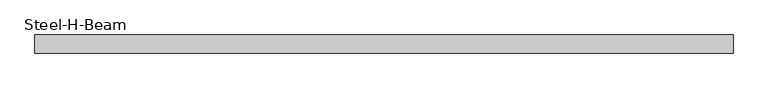
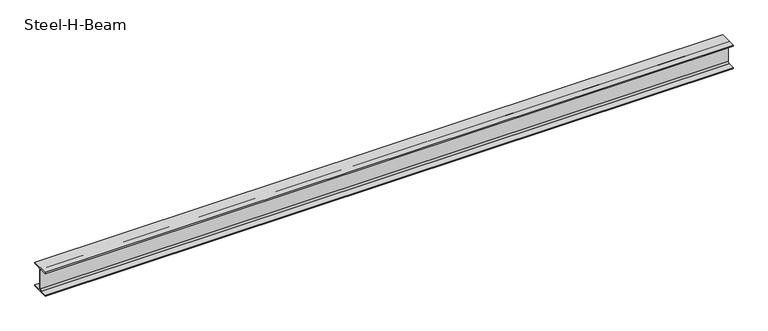
"""IFC4 building model written with IfcOpenShell, lengths in millimetres: beam geometry, Steel-H-Beam : BM121_H-244×175x7x11."""

import ifcopenshell
import ifcopenshell.guid

model = None  # the IFC model being written
_history = None  # IfcOwnerHistory: only IFC2X3 demands one
_inside = {}  # id of a spatial element -> (the spatial element, [elements in it])
_under = {}  # id of a project, library or spatial element -> (it, [spatial elements below it])
_declared = {}  # id of a project -> (the project, [libraries it declares])
_typed = {}  # id of a type object -> (the type object, [elements of that type])
_made_of = {}  # id of a material, layer set ... -> (it, [elements and type objects made of it])


def new_model(schema):
    """Start an empty IFC model of exactly this schema.

    Asked for "IFC4X3", IfcOpenShell would pick the latest addendum, in which some entities
    have other attributes; the version numbers below select the first issue.
    IFC2X3 requires an IfcOwnerHistory on every rooted entity: one is made here for all.
    """
    global model, _history
    if schema == "IFC4X3":
        model = ifcopenshell.file(schema_version=(4, 3, 0, 0))
    else:
        model = ifcopenshell.file(schema=schema)
    _inside.clear()
    _under.clear()
    _declared.clear()
    _typed.clear()
    _made_of.clear()
    _history = None
    if model.schema == "IFC2X3":
        org = make("IfcOrganization", Name="unknown")
        user = make(
            "IfcPersonAndOrganization",
            ThePerson=make("IfcPerson", FamilyName="unknown"),
            TheOrganization=org,
        )
        app = make(
            "IfcApplication",
            ApplicationDeveloper=org,
            Version="unknown",
            ApplicationFullName="unknown",
            ApplicationIdentifier="unknown",
        )
        _history = make(
            "IfcOwnerHistory",
            OwningUser=user,
            OwningApplication=app,
            ChangeAction="ADDED",
            CreationDate=0,
        )
    return model


def make(cls, **values):
    """One entity of the class cls with the attributes given. An attribute that is None is left unset."""
    return model.create_entity(
        cls, **{name: value for name, value in values.items() if value is not None}
    )


def rooted(cls, **values):
    """An entity with a GlobalId (a new one), such as an element, a storey or a relation."""
    return make(cls, GlobalId=ifcopenshell.guid.new(), OwnerHistory=_history, **values)


def si_unit(unit_type, name, prefix=None):
    """IfcSIUnit, for example si_unit("LENGTHUNIT", "METRE", prefix="MILLI")."""
    return make("IfcSIUnit", UnitType=unit_type, Prefix=prefix, Name=name)


def assignment(units):
    """IfcUnitAssignment: the units of a project."""
    return None if units is None else make("IfcUnitAssignment", Units=units)


def point(xyz):
    """IfcCartesianPoint."""
    return None if xyz is None else make("IfcCartesianPoint", Coordinates=xyz)


def direction(xyz):
    """IfcDirection."""
    return None if xyz is None else make("IfcDirection", DirectionRatios=xyz)


def frame(location, z_axis=None, x_axis=None):
    """IfcAxis2Placement3D, a coordinate frame: its origin and axes. An axis left out is left unset."""
    return make(
        "IfcAxis2Placement3D",
        Location=point(location),
        Axis=direction(z_axis),
        RefDirection=direction(x_axis),
    )


def frame_2d(location, x_axis=None):
    """IfcAxis2Placement2D, a coordinate frame in the plane: its origin and x axis."""
    return make(
        "IfcAxis2Placement2D", Location=point(location), RefDirection=direction(x_axis)
    )


def origin():
    """The frame at (0, 0, 0) with its axes left unset."""
    return frame((0.0, 0.0, 0.0))


def place(relative_to, where):
    """IfcLocalPlacement: puts the frame where relative to a parent placement (None: the world)."""
    return make(
        "IfcLocalPlacement", PlacementRelTo=relative_to, RelativePlacement=where
    )


def context(
    kind, dimensions, precision=None, world=None, true_north=None, identifier=None
):
    """IfcGeometricRepresentationContext, for example the 3D "Model" context."""
    return make(
        "IfcGeometricRepresentationContext",
        ContextIdentifier=identifier,
        ContextType=kind,
        CoordinateSpaceDimension=dimensions,
        Precision=precision,
        WorldCoordinateSystem=world,
        TrueNorth=true_north,
    )


def project(units=None, contexts=None):
    """IfcProject with its units and contexts."""
    return rooted(
        "IfcProject",
        Name="project",
        RepresentationContexts=contexts,
        UnitsInContext=assignment(units),
    )


def spatial(cls, under=None, at=None, **own):
    """A site, building, storey or space (cls), placed at a placement, below another one or the project."""
    s = rooted(cls, ObjectPlacement=at, **own)
    if under is not None:
        _under.setdefault(under.id(), (under, []))[1].append(s)
    return s


def polyline(points):
    """IfcPolyline through the points."""
    return make("IfcPolyline", Points=[point(p) for p in points])


def circle_curve(where, radius):
    """IfcCircle in the frame where."""
    return make("IfcCircle", Position=where, Radius=radius)


def trimmed(basis, trim1, trim2, sense, master):
    """IfcTrimmedCurve: the piece of a basis curve between two trims."""
    return make(
        "IfcTrimmedCurve",
        BasisCurve=basis,
        Trim1=trim1,
        Trim2=trim2,
        SenseAgreement=sense,
        MasterRepresentation=master,
    )


def segment(curve, same_sense, transition):
    """IfcCompositeCurveSegment."""
    return make(
        "IfcCompositeCurveSegment",
        Transition=transition,
        SameSense=same_sense,
        ParentCurve=curve,
    )


def composite_curve(segments, self_intersect=None):
    """IfcCompositeCurve: segments joined end to end."""
    return make("IfcCompositeCurve", Segments=segments, SelfIntersect=self_intersect)


def outline(outer, holes=None, kind="AREA"):
    """IfcArbitraryClosedProfileDef: a profile drawn as a closed curve; with holes, ...WithVoids."""
    if holes is None:
        return make("IfcArbitraryClosedProfileDef", ProfileType=kind, OuterCurve=outer)
    return make(
        "IfcArbitraryProfileDefWithVoids",
        ProfileType=kind,
        OuterCurve=outer,
        InnerCurves=holes,
    )


def extrude(swept, where, along, depth):
    """IfcExtrudedAreaSolid: the profile swept, set in the frame where, extruded along a direction by depth."""
    return make(
        "IfcExtrudedAreaSolid",
        SweptArea=swept,
        Position=where,
        ExtrudedDirection=direction(along),
        Depth=depth,
    )


def shape(context_of_items, identifier, shape_type, items):
    """IfcShapeRepresentation: the items that make up one representation, for example the "Body"."""
    return make(
        "IfcShapeRepresentation",
        ContextOfItems=context_of_items,
        RepresentationIdentifier=identifier,
        RepresentationType=shape_type,
        Items=items,
    )


def source(mapping_origin, context_of_items, identifier, shape_type, items):
    """IfcRepresentationMap: a shape defined once, which mapped items show again and again."""
    return make(
        "IfcRepresentationMap",
        MappingOrigin=mapping_origin,
        MappedRepresentation=shape(context_of_items, identifier, shape_type, items),
    )


def transform(
    local_origin,
    x_axis=None,
    y_axis=None,
    z_axis=None,
    scale=None,
    scale2=None,
    scale3=None,
    uniform=True,
):
    """IfcCartesianTransformationOperator3D, or its non-uniform kind. x_axis, y_axis, z_axis: its Axis1, 2, 3."""
    if uniform:
        return make(
            "IfcCartesianTransformationOperator3D",
            Axis1=direction(x_axis),
            Axis2=direction(y_axis),
            LocalOrigin=point(local_origin),
            Scale=scale,
            Axis3=direction(z_axis),
        )
    return make(
        "IfcCartesianTransformationOperator3DnonUniform",
        Axis1=direction(x_axis),
        Axis2=direction(y_axis),
        LocalOrigin=point(local_origin),
        Scale=scale,
        Axis3=direction(z_axis),
        Scale2=scale2,
        Scale3=scale3,
    )


def mapped(mapping_source, mapping_target):
    """IfcMappedItem: shows the shape of a source again, moved by a transform."""
    return make(
        "IfcMappedItem", MappingSource=mapping_source, MappingTarget=mapping_target
    )


def made_of(thing, what):
    """Note that an element or type object is made of a material, layer set ...; save() writes the relation."""
    if what is not None:
        _made_of.setdefault(what.id(), (what, []))[1].append(thing)
    return thing


def element(
    cls,
    number,
    at=None,
    inside=None,
    cuts=None,
    type_object=None,
    material=None,
    context=None,
    identifier="Body",
    shape_type=None,
    held_by="IfcProductDefinitionShape",
    body=None,
    shapes=None,
    **own,
):
    """One element of the class cls, such as IfcWall. Its Tag is "e" and its number.

    at: its placement. inside: the storey or other place that contains it. cuts: it is an
    opening in that element (IfcRelVoidsElement). A single representation is given by context,
    identifier, shape_type and body (its items); several are given by shapes. held_by: the class
    of the entity that holds the representations. save() writes the other relations.
    """
    e = rooted(cls, Tag="e%d" % number, ObjectPlacement=at, **own)
    if body is not None:
        shapes = [shape(context, identifier, shape_type, body)]
    if shapes is not None:
        e.Representation = make(held_by, Representations=shapes)
    if inside is not None:
        _inside.setdefault(inside.id(), (inside, []))[1].append(e)
    if cuts is not None:
        rooted(
            "IfcRelVoidsElement", RelatingBuildingElement=cuts, RelatedOpeningElement=e
        )
    if type_object is not None:
        _typed.setdefault(type_object.id(), (type_object, []))[1].append(e)
    return made_of(e, material)


def aggregate(whole, parts):
    """IfcRelAggregates: a whole, such as a stair, and the parts it consists of."""
    return rooted("IfcRelAggregates", RelatingObject=whole, RelatedObjects=parts)


def save(model, path):
    """Write the relations noted so far, then the file.

    IfcRelAggregates (storeys below a building ...), IfcRelContainedInSpatialStructure (elements
    in a storey), IfcRelDefinesByType, IfcRelAssociatesMaterial and IfcRelDeclares: one each for
    every whole, place, type object, material and project.
    """
    for whole, parts in _under.values():
        aggregate(whole, parts)
    for where, things in _inside.values():
        rooted(
            "IfcRelContainedInSpatialStructure",
            RelatedElements=things,
            RelatingStructure=where,
        )
    for kind, things in _typed.values():
        rooted("IfcRelDefinesByType", RelatedObjects=things, RelatingType=kind)
    for what, things in _made_of.values():
        rooted("IfcRelAssociatesMaterial", RelatedObjects=things, RelatingMaterial=what)
    for by, libraries in _declared.values():
        rooted("IfcRelDeclares", RelatingContext=by, RelatedDefinitions=libraries)
    model.write(path)


def steel_h_beam_0520d745(model_context):
    return source(origin(), model_context, "Body", "SweptSolid", [
        extrude(outline(composite_curve([segment(polyline([(87.5, -111.0), (87.5, -122.0), (-87.5, -122.0), (-87.5, -111.0), (-19.5, -111.0)]), True, "CONTINUOUS"), segment(trimmed(circle_curve(frame_2d((-19.5, -95.0)), 16.0), [point((-19.5, -111.0))], [point((-3.5, -95.0))], True, "CARTESIAN"), True, "CONTINUOUS"), segment(polyline([(-3.5, -95.0), (-3.5, 95.0)]), True, "CONTINUOUS"), segment(trimmed(circle_curve(frame_2d((-19.5, 95.0)), 16.0), [point((-3.5, 95.0))], [point((-19.5, 111.0))], True, "CARTESIAN"), True, "CONTINUOUS"), segment(polyline([(-19.5, 111.0), (-87.5, 111.0), (-87.5, 122.0), (87.5, 122.0), (87.5, 111.0), (19.5, 111.0)]), True, "CONTINUOUS"), segment(trimmed(circle_curve(frame_2d((19.5, 95.0)), 16.0), [point((19.5, 111.0))], [point((3.5, 95.0))], True, "CARTESIAN"), True, "CONTINUOUS"), segment(polyline([(3.5, 95.0), (3.5, -95.0)]), True, "CONTINUOUS"), segment(trimmed(circle_curve(frame_2d((19.5, -95.0)), 16.0), [point((3.5, -95.0))], [point((19.5, -111.0))], True, "CARTESIAN"), True, "CONTINUOUS"), segment(polyline([(19.5, -111.0), (87.5, -111.0)]), True, "CONTINUOUS")], self_intersect=False)), frame((-3363.2513255, 0.0, 0.0), z_axis=(1.0, 0.0, 0.0), x_axis=(0.0, 1.0, 0.0)), (0.0, 0.0, 1.0), 6724.6),
    ])


if __name__ == "__main__":
    model = new_model("IFC4")
    model_context = context("Model", 3, world=origin())
    ifc_project = project(units=[si_unit("LENGTHUNIT", "METRE", prefix="MILLI")], contexts=[model_context])
    site = spatial("IfcSite", under=ifc_project)
    building = spatial("IfcBuilding", under=site)
    placement = place(None, origin())
    steel_h_beam_shape = steel_h_beam_0520d745(model_context)
    element("IfcBeam", 1, ObjectType="Steel-H-Beam : BM121_H-244×175x7x11", at=placement, inside=building, context=model_context, shape_type="MappedRepresentation", body=[
        mapped(steel_h_beam_shape, transform((0.0, 0.0, 0.0), x_axis=(1.0, 0.0, 0.0), y_axis=(0.0, 1.0, 0.0), z_axis=(0.0, 0.0, 1.0))),
    ])
    save(model, "model.ifc")

# Revit data of these elements
# Type "Steel-H-Beam : BM121_H-244×175x7x11"
#   Surface Area = 1.14653 m²/m
#   Section Area = 56.2375 cm²
#   Mass per Unit Length = 44.1465 kg/m
#   Length [instance default] = 3000 mm
#   B = 175 mm
#   H = 244 mm
#   r = 16 mm
#   tw = 7 mm
#   tf = 11 mm
#   hec_material4 [instance default] = none
#   hec_material3 [instance default] = none
#   hec_material2 [instance default] = none
#   hec_material1 [instance default] = none
#   Structural Material [instance default] = Steel, 45-345
#   Assembly Code = ""
# Element 1 (IfcBeam, "Steel-H-Beam : BM121_H-244×175x7x11")
#   hec_material3 = F01AC000-00002_Building/Shelter Fire Proofing Work_Intumescent Coating Type_1 hr. rating (UL 1709))
#   hec_material2 = S01AA010-00002_Main Steel Structure Fabrication Work_Shelter/Building_Steel Painting/Coating_for Fireproofed Steel Surface, Surface Preparation & Primer Coat
#   hec_material1 = S03AA028-00001_Main Steel Structure Erection Work_Shelter/Building_Medium Steel
#   Materials on its faces: "Steel, 45-345"
# Materials
#   "Steel, 45-345": class "Metal", colour RGB 189 187 185, transparency 0, Description = "Steel 345 MPa", Cost = 0
#   "F01AC000-00002_Building/Shelter Fire Proofing Work_Intumescent Coating Type_1 hr. rating (UL 1709))": class "Metal", colour RGB 255 128 128, transparency 0, Description = "Paint finished steel", W00) Work Master Code = "F01AC000-00002", W01) Work Master_Lv1 = "Building/Shelter Fire Proofing Work", W02) Work Master_Lv2 = "Intumescent Coating Type", W03) Work Master_Spec.1 = "1 hr. rating (UL 1709)", Cost = 0
#   "S01AA010-00002_Main Steel Structure Fabrication Work_Shelter/Building_Steel Painting/Coating_for Fireproofed Steel Surface, Surface Preparation & Primer Coat": class "Metal", colour RGB 120 120 120, transparency 0, Description = "Paint finished steel", W00) Work Master Code = "SS01AA010-00002", W01) Work Master_Lv1 = "Main Steel Structure Fabrication Work", W02) Work Master_Lv2 = "Shelter/Building", W03) Work Master_Spec.1 = "Steel Painting/Coating", W04) Work Master_Spec.2 = "for Fireproofed Steel Surface, Surface Preparation & Primer Coat", Cost = 0
#   "S03AA028-00001_Main Steel Structure Erection Work_Shelter/Building_Medium Steel": class "Metal", colour RGB 120 120 120, transparency 0, Comments = "(90KG/M>Weight≥30KG/M)", Description = "Structural steel 50ksi", W00) Work Master Code = "S03AA028-0001", W01) Work Master_Lv1 = "Main Steel Structure Erection Work", W02) Work Master_Lv2 = "Shelter/Building", W03) Work Master_Spec.1 = "Medium Steel (90KG/M>Weight≥30KG/M)", Cost = 0
